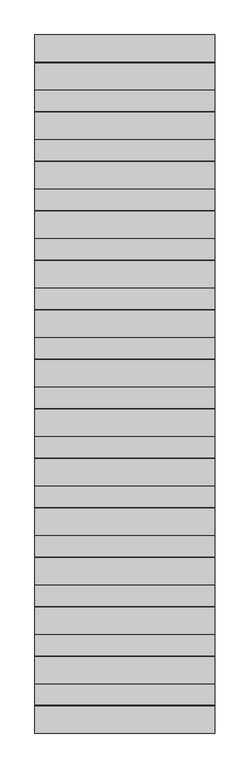
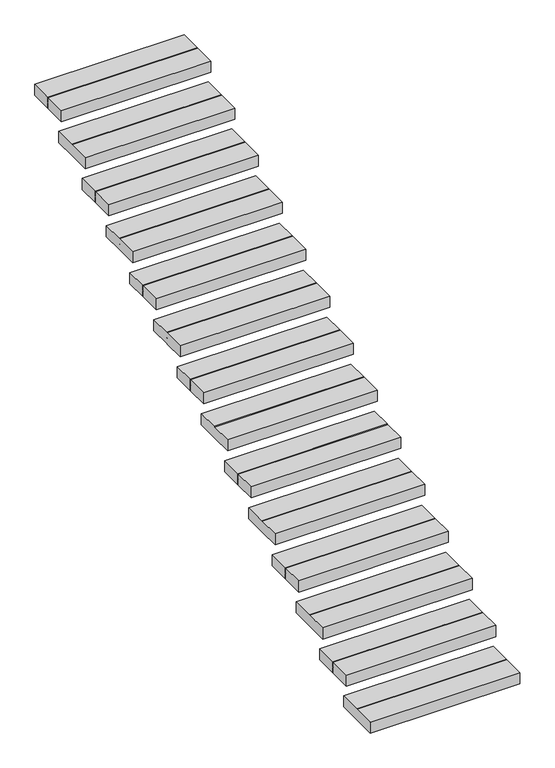
"""IFC4 building model written with IfcOpenShell, lengths in millimetres: stair flight geometry."""

import ifcopenshell
import ifcopenshell.guid

model = None  # the IFC model being written
_history = None  # IfcOwnerHistory: only IFC2X3 demands one
_inside = {}  # id of a spatial element -> (the spatial element, [elements in it])
_under = {}  # id of a project, library or spatial element -> (it, [spatial elements below it])
_declared = {}  # id of a project -> (the project, [libraries it declares])
_typed = {}  # id of a type object -> (the type object, [elements of that type])
_made_of = {}  # id of a material, layer set ... -> (it, [elements and type objects made of it])


def new_model(schema):
    """Start an empty IFC model of exactly this schema.

    Asked for "IFC4X3", IfcOpenShell would pick the latest addendum, in which some entities
    have other attributes; the version numbers below select the first issue.
    IFC2X3 requires an IfcOwnerHistory on every rooted entity: one is made here for all.
    """
    global model, _history
    if schema == "IFC4X3":
        model = ifcopenshell.file(schema_version=(4, 3, 0, 0))
    else:
        model = ifcopenshell.file(schema=schema)
    _inside.clear()
    _under.clear()
    _declared.clear()
    _typed.clear()
    _made_of.clear()
    _history = None
    if model.schema == "IFC2X3":
        org = make("IfcOrganization", Name="unknown")
        user = make(
            "IfcPersonAndOrganization",
            ThePerson=make("IfcPerson", FamilyName="unknown"),
            TheOrganization=org,
        )
        app = make(
            "IfcApplication",
            ApplicationDeveloper=org,
            Version="unknown",
            ApplicationFullName="unknown",
            ApplicationIdentifier="unknown",
        )
        _history = make(
            "IfcOwnerHistory",
            OwningUser=user,
            OwningApplication=app,
            ChangeAction="ADDED",
            CreationDate=0,
        )
    return model


def make(cls, **values):
    """One entity of the class cls with the attributes given. An attribute that is None is left unset."""
    return model.create_entity(
        cls, **{name: value for name, value in values.items() if value is not None}
    )


def rooted(cls, **values):
    """An entity with a GlobalId (a new one), such as an element, a storey or a relation."""
    return make(cls, GlobalId=ifcopenshell.guid.new(), OwnerHistory=_history, **values)


def si_unit(unit_type, name, prefix=None):
    """IfcSIUnit, for example si_unit("LENGTHUNIT", "METRE", prefix="MILLI")."""
    return make("IfcSIUnit", UnitType=unit_type, Prefix=prefix, Name=name)


def assignment(units):
    """IfcUnitAssignment: the units of a project."""
    return None if units is None else make("IfcUnitAssignment", Units=units)


def point(xyz):
    """IfcCartesianPoint."""
    return None if xyz is None else make("IfcCartesianPoint", Coordinates=xyz)


def direction(xyz):
    """IfcDirection."""
    return None if xyz is None else make("IfcDirection", DirectionRatios=xyz)


def frame(location, z_axis=None, x_axis=None):
    """IfcAxis2Placement3D, a coordinate frame: its origin and axes. An axis left out is left unset."""
    return make(
        "IfcAxis2Placement3D",
        Location=point(location),
        Axis=direction(z_axis),
        RefDirection=direction(x_axis),
    )


def origin():
    """The frame at (0, 0, 0) with its axes left unset."""
    return frame((0.0, 0.0, 0.0))


def place(relative_to, where):
    """IfcLocalPlacement: puts the frame where relative to a parent placement (None: the world)."""
    return make(
        "IfcLocalPlacement", PlacementRelTo=relative_to, RelativePlacement=where
    )


def context(
    kind, dimensions, precision=None, world=None, true_north=None, identifier=None
):
    """IfcGeometricRepresentationContext, for example the 3D "Model" context."""
    return make(
        "IfcGeometricRepresentationContext",
        ContextIdentifier=identifier,
        ContextType=kind,
        CoordinateSpaceDimension=dimensions,
        Precision=precision,
        WorldCoordinateSystem=world,
        TrueNorth=true_north,
    )


def project(units=None, contexts=None):
    """IfcProject with its units and contexts."""
    return rooted(
        "IfcProject",
        Name="project",
        RepresentationContexts=contexts,
        UnitsInContext=assignment(units),
    )


def spatial(cls, under=None, at=None, **own):
    """A site, building, storey or space (cls), placed at a placement, below another one or the project."""
    s = rooted(cls, ObjectPlacement=at, **own)
    if under is not None:
        _under.setdefault(under.id(), (under, []))[1].append(s)
    return s


def polyline(points):
    """IfcPolyline through the points."""
    return make("IfcPolyline", Points=[point(p) for p in points])


def outline(outer, holes=None, kind="AREA"):
    """IfcArbitraryClosedProfileDef: a profile drawn as a closed curve; with holes, ...WithVoids."""
    if holes is None:
        return make("IfcArbitraryClosedProfileDef", ProfileType=kind, OuterCurve=outer)
    return make(
        "IfcArbitraryProfileDefWithVoids",
        ProfileType=kind,
        OuterCurve=outer,
        InnerCurves=holes,
    )


def extrude(swept, where, along, depth):
    """IfcExtrudedAreaSolid: the profile swept, set in the frame where, extruded along a direction by depth."""
    return make(
        "IfcExtrudedAreaSolid",
        SweptArea=swept,
        Position=where,
        ExtrudedDirection=direction(along),
        Depth=depth,
    )


def shape(context_of_items, identifier, shape_type, items):
    """IfcShapeRepresentation: the items that make up one representation, for example the "Body"."""
    return make(
        "IfcShapeRepresentation",
        ContextOfItems=context_of_items,
        RepresentationIdentifier=identifier,
        RepresentationType=shape_type,
        Items=items,
    )


def source(mapping_origin, context_of_items, identifier, shape_type, items):
    """IfcRepresentationMap: a shape defined once, which mapped items show again and again."""
    return make(
        "IfcRepresentationMap",
        MappingOrigin=mapping_origin,
        MappedRepresentation=shape(context_of_items, identifier, shape_type, items),
    )


def transform(
    local_origin,
    x_axis=None,
    y_axis=None,
    z_axis=None,
    scale=None,
    scale2=None,
    scale3=None,
    uniform=True,
):
    """IfcCartesianTransformationOperator3D, or its non-uniform kind. x_axis, y_axis, z_axis: its Axis1, 2, 3."""
    if uniform:
        return make(
            "IfcCartesianTransformationOperator3D",
            Axis1=direction(x_axis),
            Axis2=direction(y_axis),
            LocalOrigin=point(local_origin),
            Scale=scale,
            Axis3=direction(z_axis),
        )
    return make(
        "IfcCartesianTransformationOperator3DnonUniform",
        Axis1=direction(x_axis),
        Axis2=direction(y_axis),
        LocalOrigin=point(local_origin),
        Scale=scale,
        Axis3=direction(z_axis),
        Scale2=scale2,
        Scale3=scale3,
    )


def mapped(mapping_source, mapping_target):
    """IfcMappedItem: shows the shape of a source again, moved by a transform."""
    return make(
        "IfcMappedItem", MappingSource=mapping_source, MappingTarget=mapping_target
    )


def made_of(thing, what):
    """Note that an element or type object is made of a material, layer set ...; save() writes the relation."""
    if what is not None:
        _made_of.setdefault(what.id(), (what, []))[1].append(thing)
    return thing


def element(
    cls,
    number,
    at=None,
    inside=None,
    cuts=None,
    type_object=None,
    material=None,
    context=None,
    identifier="Body",
    shape_type=None,
    held_by="IfcProductDefinitionShape",
    body=None,
    shapes=None,
    **own,
):
    """One element of the class cls, such as IfcWall. Its Tag is "e" and its number.

    at: its placement. inside: the storey or other place that contains it. cuts: it is an
    opening in that element (IfcRelVoidsElement). A single representation is given by context,
    identifier, shape_type and body (its items); several are given by shapes. held_by: the class
    of the entity that holds the representations. save() writes the other relations.
    """
    e = rooted(cls, Tag="e%d" % number, ObjectPlacement=at, **own)
    if body is not None:
        shapes = [shape(context, identifier, shape_type, body)]
    if shapes is not None:
        e.Representation = make(held_by, Representations=shapes)
    if inside is not None:
        _inside.setdefault(inside.id(), (inside, []))[1].append(e)
    if cuts is not None:
        rooted(
            "IfcRelVoidsElement", RelatingBuildingElement=cuts, RelatedOpeningElement=e
        )
    if type_object is not None:
        _typed.setdefault(type_object.id(), (type_object, []))[1].append(e)
    return made_of(e, material)


def aggregate(whole, parts):
    """IfcRelAggregates: a whole, such as a stair, and the parts it consists of."""
    return rooted("IfcRelAggregates", RelatingObject=whole, RelatedObjects=parts)


def save(model, path):
    """Write the relations noted so far, then the file.

    IfcRelAggregates (storeys below a building ...), IfcRelContainedInSpatialStructure (elements
    in a storey), IfcRelDefinesByType, IfcRelAssociatesMaterial and IfcRelDeclares: one each for
    every whole, place, type object, material and project.
    """
    for whole, parts in _under.values():
        aggregate(whole, parts)
    for where, things in _inside.values():
        rooted(
            "IfcRelContainedInSpatialStructure",
            RelatedElements=things,
            RelatingStructure=where,
        )
    for kind, things in _typed.values():
        rooted("IfcRelDefinesByType", RelatedObjects=things, RelatingType=kind)
    for what, things in _made_of.values():
        rooted("IfcRelAssociatesMaterial", RelatedObjects=things, RelatingMaterial=what)
    for by, libraries in _declared.values():
        rooted("IfcRelDeclares", RelatingContext=by, RelatedDefinitions=libraries)
    model.write(path)


def stair_flight_92b4aae8(model_context):
    return source(origin(), model_context, "Body", "SweptSolid", [
        extrude(outline(polyline([(31079.7618167, 264198.1), (31079.7618167, 264161.5875), (31086.1118167, 264161.5875), (31086.1118167, 264198.1), (31238.5118167, 264198.1), (31238.5118167, 264118.725), (31086.1118167, 264118.725), (31086.1118167, 264155.2375), (31079.7618167, 264155.2375), (31079.7618167, 264118.725), (30927.3618167, 264118.725), (30927.3618167, 264198.1), (31079.7618167, 264198.1)])), frame((32143.6965778, 0.0, 0.0), z_axis=(1.0, 0.0, 0.0), x_axis=(0.0, 1.0, 0.0)), (0.0, 0.0, 1.0), 1016.0),
        extrude(outline(polyline([(31359.1618167, 264366.375), (31359.1618167, 264329.8625), (31365.5118167, 264329.8625), (31365.5118167, 264366.375), (31517.9118167, 264366.375), (31517.9118167, 264287.0), (31365.5118167, 264287.0), (31365.5118167, 264323.5125), (31359.1618167, 264323.5125), (31359.1618167, 264287.0), (31206.7618167, 264287.0), (31206.7618167, 264366.375), (31359.1618167, 264366.375)])), frame((32143.6965778, 0.0, 0.0), z_axis=(1.0, 0.0, 0.0), x_axis=(0.0, 1.0, 0.0)), (0.0, 0.0, 1.0), 1016.0),
        extrude(outline(polyline([(31638.5618167, 264534.65), (31638.5618167, 264498.1375), (31644.9118167, 264498.1375), (31644.9118167, 264534.65), (31797.3118167, 264534.65), (31797.3118167, 264455.275), (31644.9118167, 264455.275), (31644.9118167, 264491.7875), (31638.5618167, 264491.7875), (31638.5618167, 264455.275), (31486.1618167, 264455.275), (31486.1618167, 264534.65), (31638.5618167, 264534.65)])), frame((32143.6965778, 0.0, 0.0), z_axis=(1.0, 0.0, 0.0), x_axis=(0.0, 1.0, 0.0)), (0.0, 0.0, 1.0), 1016.0),
        extrude(outline(polyline([(31917.9618167, 264702.925), (31917.9618167, 264666.4125), (31924.3118167, 264666.4125), (31924.3118167, 264702.925), (32076.7118167, 264702.925), (32076.7118167, 264623.55), (31924.3118167, 264623.55), (31924.3118167, 264660.0625), (31917.9618167, 264660.0625), (31917.9618167, 264623.55), (31765.5618167, 264623.55), (31765.5618167, 264702.925), (31917.9618167, 264702.925)])), frame((32143.6965778, 0.0, 0.0), z_axis=(1.0, 0.0, 0.0), x_axis=(0.0, 1.0, 0.0)), (0.0, 0.0, 1.0), 1016.0),
        extrude(outline(polyline([(32197.3618167, 264871.2), (32197.3618167, 264834.6875), (32203.7118167, 264834.6875), (32203.7118167, 264871.2), (32356.1118167, 264871.2), (32356.1118167, 264791.825), (32203.7118167, 264791.825), (32203.7118167, 264828.3375), (32197.3618167, 264828.3375), (32197.3618167, 264791.825), (32044.9618167, 264791.825), (32044.9618167, 264871.2), (32197.3618167, 264871.2)])), frame((32143.6965778, 0.0, 0.0), z_axis=(1.0, 0.0, 0.0), x_axis=(0.0, 1.0, 0.0)), (0.0, 0.0, 1.0), 1016.0),
        extrude(outline(polyline([(32476.7618167, 265039.475), (32476.7618167, 265002.9625), (32483.1118167, 265002.9625), (32483.1118167, 265039.475), (32635.5118167, 265039.475), (32635.5118167, 264960.1), (32483.1118167, 264960.1), (32483.1118167, 264996.6125), (32476.7618167, 264996.6125), (32476.7618167, 264960.1), (32324.3618167, 264960.1), (32324.3618167, 265039.475), (32476.7618167, 265039.475)])), frame((32143.6965778, 0.0, 0.0), z_axis=(1.0, 0.0, 0.0), x_axis=(0.0, 1.0, 0.0)), (0.0, 0.0, 1.0), 1016.0),
        extrude(outline(polyline([(32756.1618167, 265207.75), (32756.1618167, 265171.2375), (32762.5118167, 265171.2375), (32762.5118167, 265207.75), (32914.9118167, 265207.75), (32914.9118167, 265128.375), (32762.5118167, 265128.375), (32762.5118167, 265164.8875), (32756.1618167, 265164.8875), (32756.1618167, 265128.375), (32603.7618167, 265128.375), (32603.7618167, 265207.75), (32756.1618167, 265207.75)])), frame((32143.6965778, 0.0, 0.0), z_axis=(1.0, 0.0, 0.0), x_axis=(0.0, 1.0, 0.0)), (0.0, 0.0, 1.0), 1016.0),
        extrude(outline(polyline([(33035.5618167, 265376.025), (33035.5618167, 265339.5125), (33041.9118167, 265339.5125), (33041.9118167, 265376.025), (33194.3118167, 265376.025), (33194.3118167, 265296.65), (33041.9118167, 265296.65), (33041.9118167, 265333.1625), (33035.5618167, 265333.1625), (33035.5618167, 265296.65), (32883.1618167, 265296.65), (32883.1618167, 265376.025), (33035.5618167, 265376.025)])), frame((32143.6965778, 0.0, 0.0), z_axis=(1.0, 0.0, 0.0), x_axis=(0.0, 1.0, 0.0)), (0.0, 0.0, 1.0), 1016.0),
        extrude(outline(polyline([(33314.9618167, 265544.3), (33314.9618167, 265507.7875), (33321.3118167, 265507.7875), (33321.3118167, 265544.3), (33473.7118167, 265544.3), (33473.7118167, 265464.925), (33321.3118167, 265464.925), (33321.3118167, 265501.4375), (33314.9618167, 265501.4375), (33314.9618167, 265464.925), (33162.5618167, 265464.925), (33162.5618167, 265544.3), (33314.9618167, 265544.3)])), frame((32143.6965778, 0.0, 0.0), z_axis=(1.0, 0.0, 0.0), x_axis=(0.0, 1.0, 0.0)), (0.0, 0.0, 1.0), 1016.0),
        extrude(outline(polyline([(33594.3618167, 265712.575), (33594.3618167, 265676.0625), (33600.7118167, 265676.0625), (33600.7118167, 265712.575), (33753.1118167, 265712.575), (33753.1118167, 265633.2), (33600.7118167, 265633.2), (33600.7118167, 265669.7125), (33594.3618167, 265669.7125), (33594.3618167, 265633.2), (33441.9618167, 265633.2), (33441.9618167, 265712.575), (33594.3618167, 265712.575)])), frame((32143.6965778, 0.0, 0.0), z_axis=(1.0, 0.0, 0.0), x_axis=(0.0, 1.0, 0.0)), (0.0, 0.0, 1.0), 1016.0),
        extrude(outline(polyline([(33873.7618167, 265880.85), (33873.7618167, 265844.3375), (33880.1118167, 265844.3375), (33880.1118167, 265880.85), (34032.5118167, 265880.85), (34032.5118167, 265801.475), (33880.1118167, 265801.475), (33880.1118167, 265837.9875), (33873.7618167, 265837.9875), (33873.7618167, 265801.475), (33721.3618167, 265801.475), (33721.3618167, 265880.85), (33873.7618167, 265880.85)])), frame((32143.6965778, 0.0, 0.0), z_axis=(1.0, 0.0, 0.0), x_axis=(0.0, 1.0, 0.0)), (0.0, 0.0, 1.0), 1016.0),
        extrude(outline(polyline([(34153.1618167, 266049.125), (34153.1618167, 266012.6125), (34159.5118167, 266012.6125), (34159.5118167, 266049.125), (34311.9118167, 266049.125), (34311.9118167, 265969.75), (34159.5118167, 265969.75), (34159.5118167, 266006.2625), (34153.1618167, 266006.2625), (34153.1618167, 265969.75), (34000.7618167, 265969.75), (34000.7618167, 266049.125), (34153.1618167, 266049.125)])), frame((32143.6965778, 0.0, 0.0), z_axis=(1.0, 0.0, 0.0), x_axis=(0.0, 1.0, 0.0)), (0.0, 0.0, 1.0), 1016.0),
        extrude(outline(polyline([(34432.5618167, 266217.4), (34432.5618167, 266180.8875), (34438.9118167, 266180.8875), (34438.9118167, 266217.4), (34591.3118167, 266217.4), (34591.3118167, 266138.025), (34438.9118167, 266138.025), (34438.9118167, 266174.5375), (34432.5618167, 266174.5375), (34432.5618167, 266138.025), (34280.1618167, 266138.025), (34280.1618167, 266217.4), (34432.5618167, 266217.4)])), frame((32143.6965778, 0.0, 0.0), z_axis=(1.0, 0.0, 0.0), x_axis=(0.0, 1.0, 0.0)), (0.0, 0.0, 1.0), 1016.0),
        extrude(outline(polyline([(34711.9618167, 266385.675), (34711.9618167, 266349.1625), (34718.3118167, 266349.1625), (34718.3118167, 266385.675), (34870.7118167, 266385.675), (34870.7118167, 266306.3), (34718.3118167, 266306.3), (34718.3118167, 266342.8125), (34711.9618167, 266342.8125), (34711.9618167, 266306.3), (34559.5618167, 266306.3), (34559.5618167, 266385.675), (34711.9618167, 266385.675)])), frame((32143.6965778, 0.0, 0.0), z_axis=(1.0, 0.0, 0.0), x_axis=(0.0, 1.0, 0.0)), (0.0, 0.0, 1.0), 1016.0),
    ])


if __name__ == "__main__":
    model = new_model("IFC4")
    model_context = context("Model", 3, world=origin())
    ifc_project = project(units=[si_unit("LENGTHUNIT", "METRE", prefix="MILLI")], contexts=[model_context])
    site = spatial("IfcSite", under=ifc_project)
    building = spatial("IfcBuilding", under=site)
    placement = place(None, origin())
    stair_flight_shape = stair_flight_92b4aae8(model_context)
    element("IfcStairFlight", 1, at=placement, inside=building, context=model_context, shape_type="MappedRepresentation", body=[
        mapped(stair_flight_shape, transform((0.0, 0.0, 0.0), x_axis=(1.0, 0.0, 0.0), y_axis=(0.0, 1.0, 0.0), z_axis=(0.0, 0.0, 1.0))),
    ])
    save(model, "model.ifc")

# Revit data of these elements
# Element 1 (IfcStairFlight)
#   Materials on its faces: "TREAD: (3) TREATED 4X4"
# Materials
#   "TREAD: (3) TREATED 4X4": class "Wood", colour RGB 164 134 123, transparency 0, Description = "Pinus Echinata", Cost = 0
